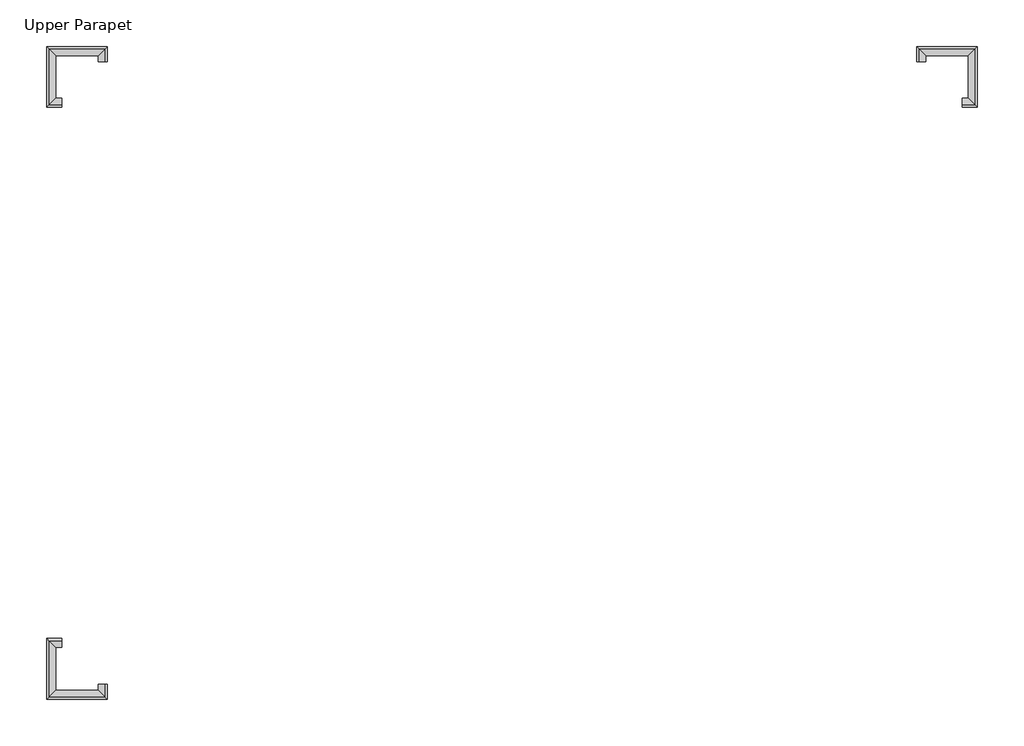
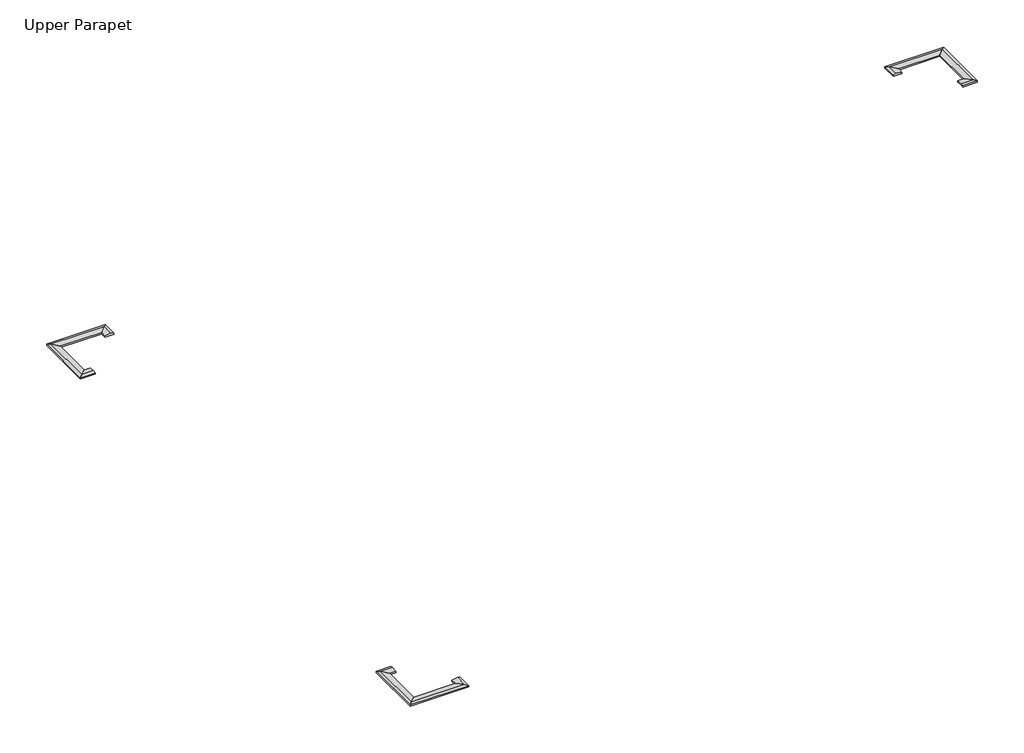
# One storey: 12 proxies.
"""IFC4 building model written with IfcOpenShell, lengths in millimetres."""

import ifcopenshell
import ifcopenshell.guid

model = None  # the IFC model being written
_history = None  # IfcOwnerHistory: only IFC2X3 demands one
_inside = {}  # id of a spatial element -> (the spatial element, [elements in it])
_under = {}  # id of a project, library or spatial element -> (it, [spatial elements below it])
_declared = {}  # id of a project -> (the project, [libraries it declares])
_typed = {}  # id of a type object -> (the type object, [elements of that type])
_made_of = {}  # id of a material, layer set ... -> (it, [elements and type objects made of it])


def new_model(schema):
    """Start an empty IFC model of exactly this schema.

    Asked for "IFC4X3", IfcOpenShell would pick the latest addendum, in which some entities
    have other attributes; the version numbers below select the first issue.
    IFC2X3 requires an IfcOwnerHistory on every rooted entity: one is made here for all.
    """
    global model, _history
    if schema == "IFC4X3":
        model = ifcopenshell.file(schema_version=(4, 3, 0, 0))
    else:
        model = ifcopenshell.file(schema=schema)
    _inside.clear()
    _under.clear()
    _declared.clear()
    _typed.clear()
    _made_of.clear()
    _history = None
    if model.schema == "IFC2X3":
        org = make("IfcOrganization", Name="unknown")
        user = make(
            "IfcPersonAndOrganization",
            ThePerson=make("IfcPerson", FamilyName="unknown"),
            TheOrganization=org,
        )
        app = make(
            "IfcApplication",
            ApplicationDeveloper=org,
            Version="unknown",
            ApplicationFullName="unknown",
            ApplicationIdentifier="unknown",
        )
        _history = make(
            "IfcOwnerHistory",
            OwningUser=user,
            OwningApplication=app,
            ChangeAction="ADDED",
            CreationDate=0,
        )
    return model


def make(cls, **values):
    """One entity of the class cls with the attributes given. An attribute that is None is left unset."""
    return model.create_entity(
        cls, **{name: value for name, value in values.items() if value is not None}
    )


def rooted(cls, **values):
    """An entity with a GlobalId (a new one), such as an element, a storey or a relation."""
    return make(cls, GlobalId=ifcopenshell.guid.new(), OwnerHistory=_history, **values)


def si_unit(unit_type, name, prefix=None):
    """IfcSIUnit, for example si_unit("LENGTHUNIT", "METRE", prefix="MILLI")."""
    return make("IfcSIUnit", UnitType=unit_type, Prefix=prefix, Name=name)


def assignment(units):
    """IfcUnitAssignment: the units of a project."""
    return None if units is None else make("IfcUnitAssignment", Units=units)


def point(xyz):
    """IfcCartesianPoint."""
    return None if xyz is None else make("IfcCartesianPoint", Coordinates=xyz)


def direction(xyz):
    """IfcDirection."""
    return None if xyz is None else make("IfcDirection", DirectionRatios=xyz)


def frame(location, z_axis=None, x_axis=None):
    """IfcAxis2Placement3D, a coordinate frame: its origin and axes. An axis left out is left unset."""
    return make(
        "IfcAxis2Placement3D",
        Location=point(location),
        Axis=direction(z_axis),
        RefDirection=direction(x_axis),
    )


def origin():
    """The frame at (0, 0, 0) with its axes left unset."""
    return frame((0.0, 0.0, 0.0))


def place(relative_to, where):
    """IfcLocalPlacement: puts the frame where relative to a parent placement (None: the world)."""
    return make(
        "IfcLocalPlacement", PlacementRelTo=relative_to, RelativePlacement=where
    )


def context(
    kind, dimensions, precision=None, world=None, true_north=None, identifier=None
):
    """IfcGeometricRepresentationContext, for example the 3D "Model" context."""
    return make(
        "IfcGeometricRepresentationContext",
        ContextIdentifier=identifier,
        ContextType=kind,
        CoordinateSpaceDimension=dimensions,
        Precision=precision,
        WorldCoordinateSystem=world,
        TrueNorth=true_north,
    )


def project(units=None, contexts=None):
    """IfcProject with its units and contexts."""
    return rooted(
        "IfcProject",
        Name="project",
        RepresentationContexts=contexts,
        UnitsInContext=assignment(units),
    )


def spatial(cls, under=None, at=None, **own):
    """A site, building, storey or space (cls), placed at a placement, below another one or the project."""
    s = rooted(cls, ObjectPlacement=at, **own)
    if under is not None:
        _under.setdefault(under.id(), (under, []))[1].append(s)
    return s


def faces_of(points, faces, orient=None, outer=None):
    """IfcFace entities. A face is a list of loops; a loop is a list of indices into points, from 0.

    orient and outer hold one flag for each loop. By default every Orientation is true, the
    first loop of a face is its IfcFaceOuterBound and the others are IfcFaceBound.
    """
    made = []
    for i, loops in enumerate(faces):
        bounds = []
        for j, loop in enumerate(loops):
            is_outer = j == 0 if outer is None else outer[i][j]
            bounds.append(
                make(
                    "IfcFaceOuterBound" if is_outer else "IfcFaceBound",
                    Bound=make("IfcPolyLoop", Polygon=[points[k] for k in loop]),
                    Orientation=True if orient is None else orient[i][j],
                )
            )
        made.append(make("IfcFace", Bounds=bounds))
    return made


def faceted_brep(points, faces, orient=None, outer=None, voids=None):
    """IfcFacetedBrep: a solid bounded by flat faces; with voids (closed shells), ...WithVoids."""
    shared = [point(p) for p in points]
    hull = make("IfcClosedShell", CfsFaces=faces_of(shared, faces, orient, outer))
    if voids is None:
        return make("IfcFacetedBrep", Outer=hull)
    return make(
        "IfcFacetedBrepWithVoids",
        Outer=hull,
        Voids=[
            make(cls, CfsFaces=faces_of(shared, fs, o, b)) for cls, fs, o, b in voids
        ],
    )


def shape(context_of_items, identifier, shape_type, items):
    """IfcShapeRepresentation: the items that make up one representation, for example the "Body"."""
    return make(
        "IfcShapeRepresentation",
        ContextOfItems=context_of_items,
        RepresentationIdentifier=identifier,
        RepresentationType=shape_type,
        Items=items,
    )


def made_of(thing, what):
    """Note that an element or type object is made of a material, layer set ...; save() writes the relation."""
    if what is not None:
        _made_of.setdefault(what.id(), (what, []))[1].append(thing)
    return thing


def element(
    cls,
    number,
    at=None,
    inside=None,
    cuts=None,
    type_object=None,
    material=None,
    context=None,
    identifier="Body",
    shape_type=None,
    held_by="IfcProductDefinitionShape",
    body=None,
    shapes=None,
    **own,
):
    """One element of the class cls, such as IfcWall. Its Tag is "e" and its number.

    at: its placement. inside: the storey or other place that contains it. cuts: it is an
    opening in that element (IfcRelVoidsElement). A single representation is given by context,
    identifier, shape_type and body (its items); several are given by shapes. held_by: the class
    of the entity that holds the representations. save() writes the other relations.
    """
    e = rooted(cls, Tag="e%d" % number, ObjectPlacement=at, **own)
    if body is not None:
        shapes = [shape(context, identifier, shape_type, body)]
    if shapes is not None:
        e.Representation = make(held_by, Representations=shapes)
    if inside is not None:
        _inside.setdefault(inside.id(), (inside, []))[1].append(e)
    if cuts is not None:
        rooted(
            "IfcRelVoidsElement", RelatingBuildingElement=cuts, RelatedOpeningElement=e
        )
    if type_object is not None:
        _typed.setdefault(type_object.id(), (type_object, []))[1].append(e)
    return made_of(e, material)


def aggregate(whole, parts):
    """IfcRelAggregates: a whole, such as a stair, and the parts it consists of."""
    return rooted("IfcRelAggregates", RelatingObject=whole, RelatedObjects=parts)


def save(model, path):
    """Write the relations noted so far, then the file.

    IfcRelAggregates (storeys below a building ...), IfcRelContainedInSpatialStructure (elements
    in a storey), IfcRelDefinesByType, IfcRelAssociatesMaterial and IfcRelDeclares: one each for
    every whole, place, type object, material and project.
    """
    for whole, parts in _under.values():
        aggregate(whole, parts)
    for where, things in _inside.values():
        rooted(
            "IfcRelContainedInSpatialStructure",
            RelatedElements=things,
            RelatingStructure=where,
        )
    for kind, things in _typed.values():
        rooted("IfcRelDefinesByType", RelatedObjects=things, RelatingType=kind)
    for what, things in _made_of.values():
        rooted("IfcRelAssociatesMaterial", RelatedObjects=things, RelatingMaterial=what)
    for by, libraries in _declared.values():
        rooted("IfcRelDeclares", RelatingContext=by, RelatedDefinitions=libraries)
    model.write(path)


model = new_model("IFC4")

# Units and contexts
model_context = context("Model", 3, world=origin())
ifc_project = project(units=[si_unit("LENGTHUNIT", "METRE", prefix="MILLI")], contexts=[model_context])

# Site, building, storey
site = spatial("IfcSite", under=ifc_project)
building = spatial("IfcBuilding", under=site)
storey = spatial("IfcBuildingStorey", under=building, Name="Upper Parapet", Elevation=7924.8)

# Proxies
placement = place(None, origin())
element("IfcBuildingElementProxy", 1, Name="Wall Sweeps", at=placement, inside=storey, context=model_context, shape_type="Brep", body=[
    faceted_brep([(-20412.8727721, 13993.4436943, 7988.3), (-20412.8727721, 13993.4436943, 7924.8), (-20384.2977721, 13993.4436943, 7924.8), (-20031.8727721, 13993.4436943, 7924.8), (-20006.4727721, 13993.4436943, 7924.8), (-20006.4727721, 13993.4436943, 7988.3), (-20133.4727721, 13993.4436943, 8026.4), (-20412.8727721, 14269.6686943, 7988.3), (-20133.4727721, 14549.0686943, 8026.4), (-20006.4727721, 14676.0686943, 7988.3), (-20006.4727721, 14676.0686943, 7924.8), (-20031.8727721, 14650.6686943, 7924.8), (-20384.2977721, 14298.2436943, 7924.8), (-20412.8727721, 14269.6686943, 7924.8)], [[[0, 1, 2, 3, 4, 5, 6]], [[7, 8, 9, 10, 11, 12, 13]], [[0, 6, 8, 7]], [[6, 5, 9, 8]], [[5, 4, 10, 9]], [[4, 3, 2, 1, 13, 12, 11, 10]], [[1, 0, 7, 13]]]),
])
element("IfcBuildingElementProxy", 2, Name="Wall Sweeps", at=placement, inside=storey, context=model_context, shape_type="Brep", body=[
    faceted_brep([(-20412.8727721, 14269.6686943, 7988.3), (-20412.8727721, 14269.6686943, 7924.8), (-20384.2977721, 14298.2436943, 7924.8), (-20031.8727721, 14650.6686943, 7924.8), (-20006.4727721, 14676.0686943, 7924.8), (-20006.4727721, 14676.0686943, 7988.3), (-20133.4727721, 14549.0686943, 8026.4), (-22343.2727721, 14269.6686943, 7988.3), (-22622.6727721, 14549.0686943, 8026.4), (-22749.6727721, 14676.0686943, 7988.3), (-22749.6727721, 14676.0686943, 7924.8), (-22724.2727721, 14650.6686943, 7924.8), (-22371.8477721, 14298.2436943, 7924.8), (-22343.2727721, 14269.6686943, 7924.8)], [[[0, 1, 2, 3, 4, 5, 6]], [[7, 8, 9, 10, 11, 12, 13]], [[0, 6, 8, 7]], [[6, 5, 9, 8]], [[5, 4, 10, 9]], [[4, 3, 2, 1, 13, 12, 11, 10]], [[1, 0, 7, 13]]]),
])
element("IfcBuildingElementProxy", 3, Name="Wall Sweeps", at=placement, inside=storey, context=model_context, shape_type="Brep", body=[
    faceted_brep([(-22343.2727721, 14269.6686943, 7988.3), (-22343.2727721, 14269.6686943, 7924.8), (-22371.8477721, 14298.2436943, 7924.8), (-22724.2727721, 14650.6686943, 7924.8), (-22749.6727721, 14676.0686943, 7924.8), (-22749.6727721, 14676.0686943, 7988.3), (-22622.6727721, 14549.0686943, 8026.4), (-22343.2727721, 12339.2686943, 7988.3), (-22622.6727721, 12059.8686943, 8026.4), (-22749.6727721, 11932.8686943, 7988.3), (-22749.6727721, 11932.8686943, 7924.8), (-22724.2727721, 11958.2686943, 7924.8), (-22371.8477721, 12310.6936943, 7924.8), (-22343.2727721, 12339.2686943, 7924.8)], [[[0, 1, 2, 3, 4, 5, 6]], [[7, 8, 9, 10, 11, 12, 13]], [[0, 6, 8, 7]], [[6, 5, 9, 8]], [[5, 4, 10, 9]], [[4, 3, 2, 1, 13, 12, 11, 10]], [[1, 0, 7, 13]]]),
])
element("IfcBuildingElementProxy", 4, Name="Wall Sweeps", at=placement, inside=storey, context=model_context, shape_type="Brep", body=[
    faceted_brep([(-22343.2727721, 12339.2686943, 7988.3), (-22343.2727721, 12339.2686943, 7924.8), (-22371.8477721, 12310.6936943, 7924.8), (-22724.2727721, 11958.2686943, 7924.8), (-22749.6727721, 11932.8686943, 7924.8), (-22749.6727721, 11932.8686943, 7988.3), (-22622.6727721, 12059.8686943, 8026.4), (-22067.0477721, 12339.2686943, 7988.3), (-22067.0477721, 12059.8686943, 8026.4), (-22067.0477721, 11932.8686943, 7988.3), (-22067.0477721, 11932.8686943, 7924.8), (-22067.0477721, 11958.2686943, 7924.8), (-22067.0477721, 12310.6936943, 7924.8), (-22067.0477721, 12339.2686943, 7924.8)], [[[0, 1, 2, 3, 4, 5, 6]], [[7, 8, 9, 10, 11, 12, 13]], [[0, 6, 8, 7]], [[6, 5, 9, 8]], [[5, 4, 10, 9]], [[4, 3, 2, 1, 13, 12, 11, 10]], [[1, 0, 7, 13]]]),
])
element("IfcBuildingElementProxy", 5, Name="Wall Sweeps", at=placement, inside=storey, context=model_context, shape_type="Brep", body=[
    faceted_brep([(-20412.8727721, -14054.5063057, 7988.3), (-20133.4727721, -14054.5063057, 8026.4), (-20006.4727721, -14054.5063057, 7988.3), (-20006.4727721, -14054.5063057, 7924.8), (-20031.8727721, -14054.5063057, 7924.8), (-20384.2977721, -14054.5063057, 7924.8), (-20412.8727721, -14054.5063057, 7924.8), (-20412.8727721, -14330.7313057, 7988.3), (-20412.8727721, -14330.7313057, 7924.8), (-20384.2977721, -14359.3063057, 7924.8), (-20031.8727721, -14711.7313057, 7924.8), (-20006.4727721, -14737.1313057, 7924.8), (-20006.4727721, -14737.1313057, 7988.3), (-20133.4727721, -14610.1313057, 8026.4)], [[[0, 1, 2, 3, 4, 5, 6]], [[7, 8, 9, 10, 11, 12, 13]], [[1, 0, 7, 13]], [[2, 1, 13, 12]], [[3, 2, 12, 11]], [[6, 5, 4, 3, 11, 10, 9, 8]], [[0, 6, 8, 7]]]),
])
element("IfcBuildingElementProxy", 6, Name="Wall Sweeps", at=placement, inside=storey, context=model_context, shape_type="Brep", body=[
    faceted_brep([(-20412.8727721, -14330.7313057, 7988.3), (-20133.4727721, -14610.1313057, 8026.4), (-20006.4727721, -14737.1313057, 7988.3), (-20006.4727721, -14737.1313057, 7924.8), (-20031.8727721, -14711.7313057, 7924.8), (-20384.2977721, -14359.3063057, 7924.8), (-20412.8727721, -14330.7313057, 7924.8), (-22343.2727721, -14330.7313057, 7988.3), (-22343.2727721, -14330.7313057, 7924.8), (-22371.8477721, -14359.3063057, 7924.8), (-22724.2727721, -14711.7313057, 7924.8), (-22749.6727721, -14737.1313057, 7924.8), (-22749.6727721, -14737.1313057, 7988.3), (-22622.6727721, -14610.1313057, 8026.4)], [[[0, 1, 2, 3, 4, 5, 6]], [[7, 8, 9, 10, 11, 12, 13]], [[1, 0, 7, 13]], [[2, 1, 13, 12]], [[3, 2, 12, 11]], [[6, 5, 4, 3, 11, 10, 9, 8]], [[0, 6, 8, 7]]]),
])
element("IfcBuildingElementProxy", 7, Name="Wall Sweeps", at=placement, inside=storey, context=model_context, shape_type="Brep", body=[
    faceted_brep([(-22343.2727721, -14330.7313057, 7988.3), (-22622.6727721, -14610.1313057, 8026.4), (-22749.6727721, -14737.1313057, 7988.3), (-22749.6727721, -14737.1313057, 7924.8), (-22724.2727721, -14711.7313057, 7924.8), (-22371.8477721, -14359.3063057, 7924.8), (-22343.2727721, -14330.7313057, 7924.8), (-22343.2727721, -12400.3313057, 7988.3), (-22343.2727721, -12400.3313057, 7924.8), (-22371.8477721, -12371.7563057, 7924.8), (-22724.2727721, -12019.3313057, 7924.8), (-22749.6727721, -11993.9313057, 7924.8), (-22749.6727721, -11993.9313057, 7988.3), (-22622.6727721, -12120.9313057, 8026.4)], [[[0, 1, 2, 3, 4, 5, 6]], [[7, 8, 9, 10, 11, 12, 13]], [[1, 0, 7, 13]], [[2, 1, 13, 12]], [[3, 2, 12, 11]], [[6, 5, 4, 3, 11, 10, 9, 8]], [[0, 6, 8, 7]]]),
])
element("IfcBuildingElementProxy", 8, Name="Wall Sweeps", at=placement, inside=storey, context=model_context, shape_type="Brep", body=[
    faceted_brep([(-22343.2727721, -12400.3313057, 7988.3), (-22622.6727721, -12120.9313057, 8026.4), (-22749.6727721, -11993.9313057, 7988.3), (-22749.6727721, -11993.9313057, 7924.8), (-22724.2727721, -12019.3313057, 7924.8), (-22371.8477721, -12371.7563057, 7924.8), (-22343.2727721, -12400.3313057, 7924.8), (-22067.0477721, -12400.3313057, 7988.3), (-22067.0477721, -12400.3313057, 7924.8), (-22067.0477721, -12371.7563057, 7924.8), (-22067.0477721, -12019.3313057, 7924.8), (-22067.0477721, -11993.9313057, 7924.8), (-22067.0477721, -11993.9313057, 7988.3), (-22067.0477721, -12120.9313057, 8026.4)], [[[0, 1, 2, 3, 4, 5, 6]], [[7, 8, 9, 10, 11, 12, 13]], [[1, 0, 7, 13]], [[2, 1, 13, 12]], [[3, 2, 12, 11]], [[6, 5, 4, 3, 11, 10, 9, 8]], [[0, 6, 8, 7]]]),
])
element("IfcBuildingElementProxy", 9, Name="Wall Sweeps", at=placement, inside=storey, context=model_context, shape_type="Brep", body=[
    faceted_brep([(16823.5272279, 13993.4436943, 7988.3), (16544.1272279, 13993.4436943, 8026.4), (16417.1272279, 13993.4436943, 7988.3), (16417.1272279, 13993.4436943, 7924.8), (16442.5272279, 13993.4436943, 7924.8), (16794.9522279, 13993.4436943, 7924.8), (16823.5272279, 13993.4436943, 7924.8), (16823.5272279, 14269.6686943, 7988.3), (16823.5272279, 14269.6686943, 7924.8), (16794.9522279, 14298.2436943, 7924.8), (16442.5272279, 14650.6686943, 7924.8), (16417.1272279, 14676.0686943, 7924.8), (16417.1272279, 14676.0686943, 7988.3), (16544.1272279, 14549.0686943, 8026.4)], [[[0, 1, 2, 3, 4, 5, 6]], [[7, 8, 9, 10, 11, 12, 13]], [[1, 0, 7, 13]], [[2, 1, 13, 12]], [[3, 2, 12, 11]], [[6, 5, 4, 3, 11, 10, 9, 8]], [[0, 6, 8, 7]]]),
])
element("IfcBuildingElementProxy", 10, Name="Wall Sweeps", at=placement, inside=storey, context=model_context, shape_type="Brep", body=[
    faceted_brep([(16823.5272279, 14269.6686943, 7988.3), (16544.1272279, 14549.0686943, 8026.4), (16417.1272279, 14676.0686943, 7988.3), (16417.1272279, 14676.0686943, 7924.8), (16442.5272279, 14650.6686943, 7924.8), (16794.9522279, 14298.2436943, 7924.8), (16823.5272279, 14269.6686943, 7924.8), (18753.9272279, 14269.6686943, 7988.3), (18753.9272279, 14269.6686943, 7924.8), (18782.5022279, 14298.2436943, 7924.8), (19134.9272279, 14650.6686943, 7924.8), (19160.3272279, 14676.0686943, 7924.8), (19160.3272279, 14676.0686943, 7988.3), (19033.3272279, 14549.0686943, 8026.4)], [[[0, 1, 2, 3, 4, 5, 6]], [[7, 8, 9, 10, 11, 12, 13]], [[1, 0, 7, 13]], [[2, 1, 13, 12]], [[3, 2, 12, 11]], [[6, 5, 4, 3, 11, 10, 9, 8]], [[0, 6, 8, 7]]]),
])
element("IfcBuildingElementProxy", 11, Name="Wall Sweeps", at=placement, inside=storey, context=model_context, shape_type="Brep", body=[
    faceted_brep([(18753.9272279, 14269.6686943, 7988.3), (19033.3272279, 14549.0686943, 8026.4), (19160.3272279, 14676.0686943, 7988.3), (19160.3272279, 14676.0686943, 7924.8), (19134.9272279, 14650.6686943, 7924.8), (18782.5022279, 14298.2436943, 7924.8), (18753.9272279, 14269.6686943, 7924.8), (18753.9272279, 12339.2686943, 7988.3), (18753.9272279, 12339.2686943, 7924.8), (18782.5022279, 12310.6936943, 7924.8), (19134.9272279, 11958.2686943, 7924.8), (19160.3272279, 11932.8686943, 7924.8), (19160.3272279, 11932.8686943, 7988.3), (19033.3272279, 12059.8686943, 8026.4)], [[[0, 1, 2, 3, 4, 5, 6]], [[7, 8, 9, 10, 11, 12, 13]], [[1, 0, 7, 13]], [[2, 1, 13, 12]], [[3, 2, 12, 11]], [[6, 5, 4, 3, 11, 10, 9, 8]], [[0, 6, 8, 7]]]),
])
element("IfcBuildingElementProxy", 12, Name="Wall Sweeps", at=placement, inside=storey, context=model_context, shape_type="Brep", body=[
    faceted_brep([(18753.9272279, 12339.2686943, 7988.3), (19033.3272279, 12059.8686943, 8026.4), (19160.3272279, 11932.8686943, 7988.3), (19160.3272279, 11932.8686943, 7924.8), (19134.9272279, 11958.2686943, 7924.8), (18782.5022279, 12310.6936943, 7924.8), (18753.9272279, 12339.2686943, 7924.8), (18477.7022279, 12339.2686943, 7988.3), (18477.7022279, 12339.2686943, 7924.8), (18477.7022279, 12310.6936943, 7924.8), (18477.7022279, 11958.2686943, 7924.8), (18477.7022279, 11932.8686943, 7924.8), (18477.7022279, 11932.8686943, 7988.3), (18477.7022279, 12059.8686943, 8026.4)], [[[0, 1, 2, 3, 4, 5, 6]], [[7, 8, 9, 10, 11, 12, 13]], [[1, 0, 7, 13]], [[2, 1, 13, 12]], [[3, 2, 12, 11]], [[6, 5, 4, 3, 11, 10, 9, 8]], [[0, 6, 8, 7]]]),
])

save(model, "model.ifc")

# Revit data of these elements
# Elements 1, 2, 3, 4, 5, 6, 7, 8, 9, 10, 11, 12 (IfcBuildingElementProxy)
#   Phase Created = New Construction
#   Materials on its faces: "Precast Cap"
# Materials
#   "Precast Cap": class "Stucco", colour RGB 129 132 118, transparency 0, Cost = 0
